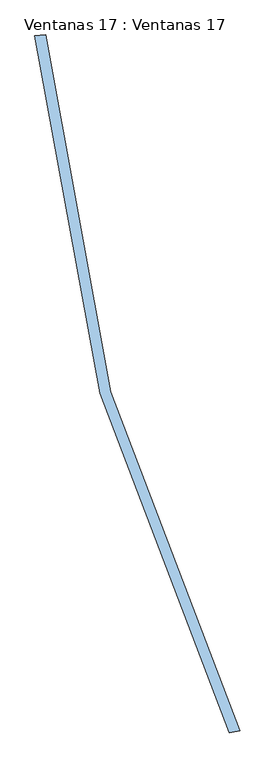
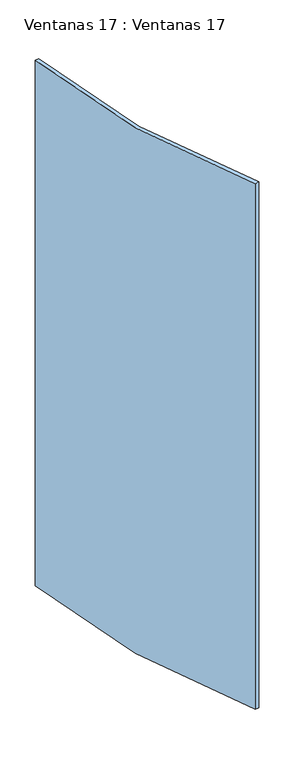
"""IFC4 building model written with IfcOpenShell, lengths in millimetres: window geometry, Ventanas 17 : Ventanas 17."""

from ifc_helpers import new_model, si_unit, point, frame, frame_2d, origin, place, context, project, spatial, polyline, circle_curve, trimmed, segment, composite_curve, outline, extrude, source, transform, mapped, element, save


def ventanas_17_ventanas_17_4045924e(model_context):
    return source(origin(), model_context, "Body", "SweptSolid", [
        extrude(outline(composite_curve([segment(polyline([(-1097.3146, 1569.0452467), (-1116.9471437, 1565.2290668)]), True, "CONTINUOUS"), segment(trimmed(circle_curve(frame_2d((2200.225295, 3194.3956515)), 3695.6483529), [point((-1116.9471437, 1565.2290668))], [point((-1480.7800815, 2865.7375214))], False, "CARTESIAN"), True, "CONTINUOUS"), segment(polyline([(-1480.7800815, 2865.7375214), (-1460.8564231, 2867.483326)]), True, "CONTINUOUS"), segment(trimmed(circle_curve(frame_2d((2178.7501221, 3186.4027676)), 3653.5524376), [point((-1460.8564231, 2867.483326))], [point((-1097.3146, 1569.0452467))], True, "CARTESIAN"), True, "CONTINUOUS")], self_intersect=False)), frame((0.0, 0.0, 6100.0), z_axis=(0.0, 0.0, 1.0), x_axis=(1.0, 0.0, 0.0)), (0.0, 0.0, 1.0), 2815.3215694),
    ])


if __name__ == "__main__":
    model = new_model("IFC4")
    model_context = context("Model", 3, world=origin())
    ifc_project = project(units=[si_unit("LENGTHUNIT", "METRE", prefix="MILLI")], contexts=[model_context])
    site = spatial("IfcSite", under=ifc_project)
    building = spatial("IfcBuilding", under=site)
    placement = place(None, origin())
    ventanas_17_ventanas_17_shape = ventanas_17_ventanas_17_4045924e(model_context)
    element("IfcWindow", 1, ObjectType="Ventanas 17 : Ventanas 17", at=placement, inside=building, context=model_context, shape_type="MappedRepresentation", body=[
        mapped(ventanas_17_ventanas_17_shape, transform((0.0, 0.0, 0.0), x_axis=(1.0, 0.0, 0.0), y_axis=(0.0, 1.0, 0.0), z_axis=(0.0, 0.0, 1.0))),
    ])
    save(model, "model.ifc")

# Revit data of these elements
# Type "Ventanas 17 : Ventanas 17"
#   Type Mark = "43"
# Element 1 (IfcWindow, "Ventanas 17 : Ventanas 17")
#   Materials on its faces: "VIDRIO"
# Materials
#   "VIDRIO": class "Genérico", colour RGB 120 120 120, transparency 0, Cost = 0
